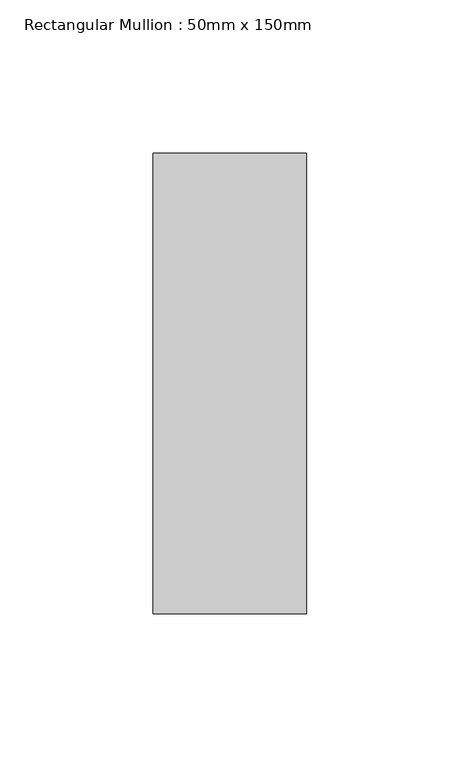
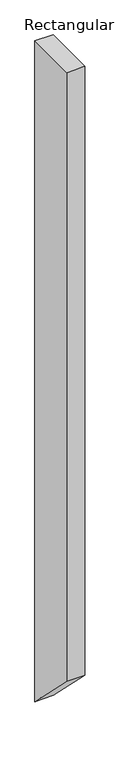
"""IFC4 building model written with IfcOpenShell, lengths in millimetres: member geometry, Rectangular Mullion : 50mm x 150mm."""

from ifc_helpers import new_model, si_unit, frame, origin, place, context, project, spatial, polyline, outline, extrude, source, transform, mapped, element, save


def rectangular_mullion_50mm_x_150mm_f6bca04a(model_context):
    return source(origin(), model_context, "Body", "SweptSolid", [
        extrude(outline(polyline([(-75.0, 0.0), (75.0, 0.0), (75.0, -1905.0000003), (-75.0, -1755.0000003), (-75.0, 0.0)])), frame((-50.0, 0.0, 0.0), z_axis=(1.0, 0.0, 0.0), x_axis=(0.0, 1.0, 0.0)), (0.0, 0.0, 1.0), 50.0),
    ])


if __name__ == "__main__":
    model = new_model("IFC4")
    model_context = context("Model", 3, world=origin())
    ifc_project = project(units=[si_unit("LENGTHUNIT", "METRE", prefix="MILLI")], contexts=[model_context])
    site = spatial("IfcSite", under=ifc_project)
    building = spatial("IfcBuilding", under=site)
    placement = place(None, origin())
    rectangular_mullion_50mm_x_150mm_shape = rectangular_mullion_50mm_x_150mm_f6bca04a(model_context)
    element("IfcMember", 1, ObjectType="Rectangular Mullion : 50mm x 150mm", at=placement, inside=building, context=model_context, shape_type="MappedRepresentation", body=[
        mapped(rectangular_mullion_50mm_x_150mm_shape, transform((0.0, 0.0, 0.0), x_axis=(1.0, 0.0, 0.0), y_axis=(0.0, 1.0, 0.0), z_axis=(0.0, 0.0, 1.0))),
    ])
    save(model, "model.ifc")

# Revit data of these elements
# Type "Rectangular Mullion : 50mm x 150mm"
#   built-in parameter 1007304 = 0.492126 (stored number, unit not read)
#   built-in parameter 1007301 = 0.082021 (stored number, unit not read)
#   built-in parameter 1007300 = 0.082021 (stored number, unit not read)
# Element 1 (IfcMember, "Rectangular Mullion : 50mm x 150mm")
#   Materials on its faces: "Aluminum"
# Materials
#   "Aluminum": class "Metal", colour RGB 244 244 244, transparency 0, Description = "Aluminum 6061", Cost = 0
